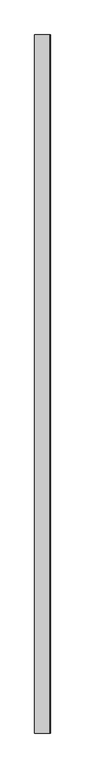
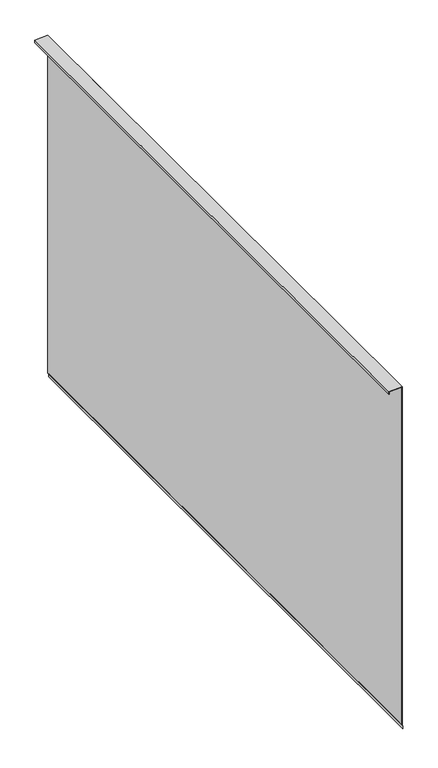
"""IFC4 building model written with IfcOpenShell, lengths in millimetres: proxy geometry, Generic Models 7:Generic Models 1:5:Generic Models 1:5 : Generic Models 7:Generic Models 1:337419:32 : Generic Models 7:Generic Models 1:5:Generic Models 1:5 : Generic Models 7:Generic Models 1:337419:311462."""

from ifc_helpers import new_model, si_unit, frame, origin, place, context, project, spatial, polyline, outline, extrude, source, transform, mapped, element, save


def generic_models_ccf0c1ab(model_context):
    return source(origin(), model_context, "Body", "SweptSolid", [
        extrude(outline(polyline([(81.1385169, 667560.8054739), (64.611433, 667572.3778627), (10.5783058, 667572.3778627), (10.5783058, 667573.9653627), (65.1119698, 667573.9653627), (81.6390538, 667562.3929739), (6180.6116872, 667562.3929739), (6168.9628216, 667340.1193767), (6125.115987, 667340.1193767), (6125.115987, 667341.7068767), (6167.4563403, 667341.7068767), (6178.9388113, 667560.8054739), (81.1385169, 667560.8054739)])), frame((0.0, -578724.4663841, 0.0), z_axis=(0.0, 1.0, 0.0), x_axis=(0.0, 0.0, 1.0)), (0.0, 0.0, 1.0), 10469.0424392),
    ])


if __name__ == "__main__":
    model = new_model("IFC4")
    model_context = context("Model", 3, world=origin())
    ifc_project = project(units=[si_unit("LENGTHUNIT", "METRE", prefix="MILLI")], contexts=[model_context])
    site = spatial("IfcSite", under=ifc_project)
    building = spatial("IfcBuilding", under=site)
    placement = place(None, origin())
    generic_models_shape = generic_models_ccf0c1ab(model_context)
    element("IfcBuildingElementProxy", 1, Name="Generic Models 7:Generic Models 1:5:Generic Models 1:5 : Generic Models 7:Generic Models 1:337419:32 : Generic Models 7:Generic Models 1:5:Generic Models 1:5 : Generic Models 7:Generic Models 1:337419:311462", ObjectType="Generic Models 7:Generic Models 1:5:Generic Models 1:5 : Generic Models 7:Generic Models 1:337419:32 : Generic Models 7:Generic Models 1:5:Generic Models 1:5 : Generic Models 7:Generic Models 1:337419:311462", at=placement, inside=building, context=model_context, shape_type="MappedRepresentation", body=[
        mapped(generic_models_shape, transform((0.0, 0.0, 0.0), x_axis=(1.0, 0.0, 0.0), y_axis=(0.0, 1.0, 0.0), z_axis=(0.0, 0.0, 1.0))),
    ])
    save(model, "model.ifc")

# Revit data of these elements
# Type "Generic Models 7:Generic Models 1:5:Generic Models 1:5 : Generic Models 7:Generic Models 1:337419:32 : Generic Models 7:Generic Models 1:5:Generic Models 1:5 : Generic Models 7:Generic Models 1:337419:311462"
#   NameOverride = "Generic Models 7:Generic Models 1:5:Generic Models 1:5 : Generic Models 7:Generic Models 1:337419:311462"
#   ObjectTypeOverride = "Generic Models 1:5 : Generic Models 7:Generic Models 1:337419"
#   Reference = "Generic Models 1"
#   Tag = "311462"
# Element 1 (IfcBuildingElementProxy, "Generic Models 7:Generic Models 1:5:Generic Models 1:5 : Generic Models 7:Generic Models 1:337419:32 : Generic Models 7:Generic Models 1:5:Generic Models 1:5 : Generic Models 7:Generic Models 1:337419:311462")
#   Materials on its faces: "UV STABLE WATER RESISTANT VAPOR PERMEABLE AIR BARRIER (WRB) - WRAP JAMBS/HEADERS - BLACK COLOR"
# Materials
#   "UV STABLE WATER RESISTANT VAPOR PERMEABLE AIR BARRIER (WRB) - WRAP JAMBS/HEADERS - BLACK COLOR": class "Generic", colour RGB 51 162 45, transparency 0, Description = "Polyethylene film membrane", Cost = 0
